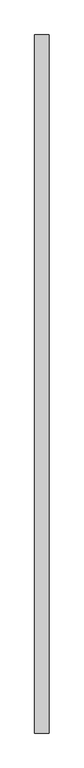
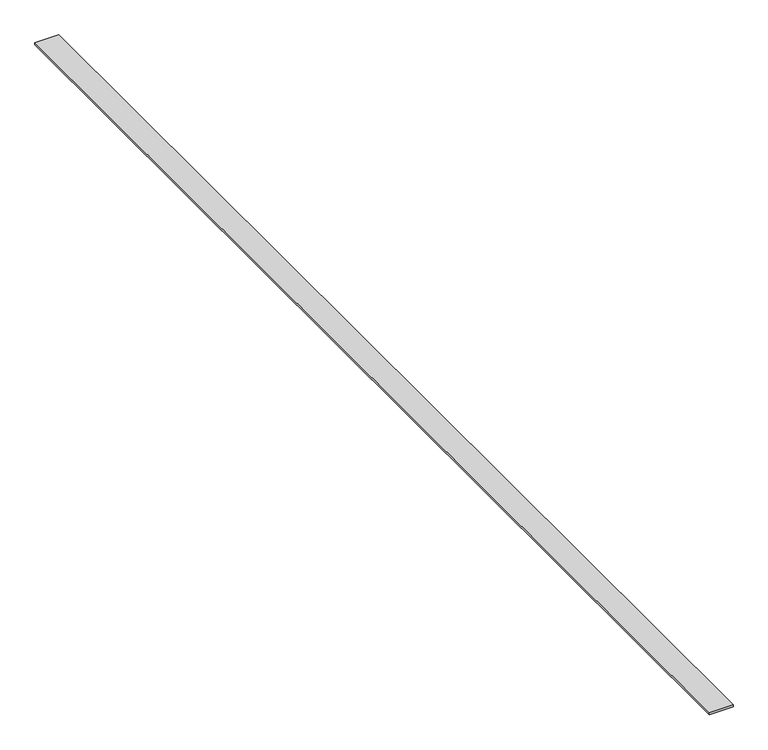
"""IFC4 building model written with IfcOpenShell, lengths in millimetres: proxy geometry, Generic Models 3:Generic Models 2:312240:Generic Models 2:312240 : Generic Models 3:Generic Models 2:312240:9 : Generic Models 3:Generic Models 2:312240:Generic Models 2:312240 : Generic Models 3:Generic Models 2:312240:300533."""

from ifc_helpers import new_model, si_unit, frame, origin, place, context, project, spatial, polyline, outline, extrude, source, transform, mapped, element, save


def generic_models_2194e599(model_context):
    return source(origin(), model_context, "Body", "SweptSolid", [
        extrude(outline(polyline([(0.0, -44.45), (0.0, 0.0), (2178.6876522, 0.0), (2178.6876522, -44.45), (0.0, -44.45)])), frame((667591.7617239, -568236.4915363, -25.4), z_axis=(-1.966712507134651e-12, 0.0, 1.0), x_axis=(0.0, 1.0, 0.0)), (0.0, 0.0, 1.0), 3.96875),
    ])


if __name__ == "__main__":
    model = new_model("IFC4")
    model_context = context("Model", 3, world=origin())
    ifc_project = project(units=[si_unit("LENGTHUNIT", "METRE", prefix="MILLI")], contexts=[model_context])
    site = spatial("IfcSite", under=ifc_project)
    building = spatial("IfcBuilding", under=site)
    placement = place(None, origin())
    generic_models_shape = generic_models_2194e599(model_context)
    element("IfcBuildingElementProxy", 1, Name="Generic Models 3:Generic Models 2:312240:Generic Models 2:312240 : Generic Models 3:Generic Models 2:312240:9 : Generic Models 3:Generic Models 2:312240:Generic Models 2:312240 : Generic Models 3:Generic Models 2:312240:300533", ObjectType="Generic Models 3:Generic Models 2:312240:Generic Models 2:312240 : Generic Models 3:Generic Models 2:312240:9 : Generic Models 3:Generic Models 2:312240:Generic Models 2:312240 : Generic Models 3:Generic Models 2:312240:300533", at=placement, inside=building, context=model_context, shape_type="MappedRepresentation", body=[
        mapped(generic_models_shape, transform((0.0, 0.0, 0.0), x_axis=(1.0, 0.0, 0.0), y_axis=(0.0, 1.0, 0.0), z_axis=(0.0, 0.0, 1.0))),
    ])
    save(model, "model.ifc")

# Revit data of these elements
# Type "Generic Models 3:Generic Models 2:312240:Generic Models 2:312240 : Generic Models 3:Generic Models 2:312240:9 : Generic Models 3:Generic Models 2:312240:Generic Models 2:312240 : Generic Models 3:Generic Models 2:312240:300533"
#   NameOverride = "Generic Models 3:Generic Models 2:312240:Generic Models 2:312240 : Generic Models 3:Generic Models 2:312240:300533"
#   ObjectTypeOverride = "Generic Models 2:312240 : Generic Models 3:Generic Models 2:312240"
#   Reference = "Generic Models 2"
#   Tag = "300533"
# Element 1 (IfcBuildingElementProxy, "Generic Models 3:Generic Models 2:312240:Generic Models 2:312240 : Generic Models 3:Generic Models 2:312240:9 : Generic Models 3:Generic Models 2:312240:Generic Models 2:312240 : Generic Models 3:Generic Models 2:312240:300533")
#   Materials on its faces: "WOOD BLOCKING - SIZE AS NECESSARY"
# Materials
#   "WOOD BLOCKING - SIZE AS NECESSARY": class "Wood", colour RGB 144 113 62, transparency 0, Description = "Pinus Echinata", Cost = 0
